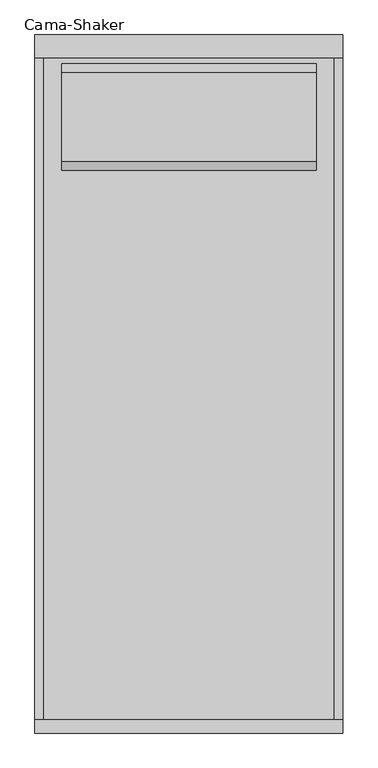
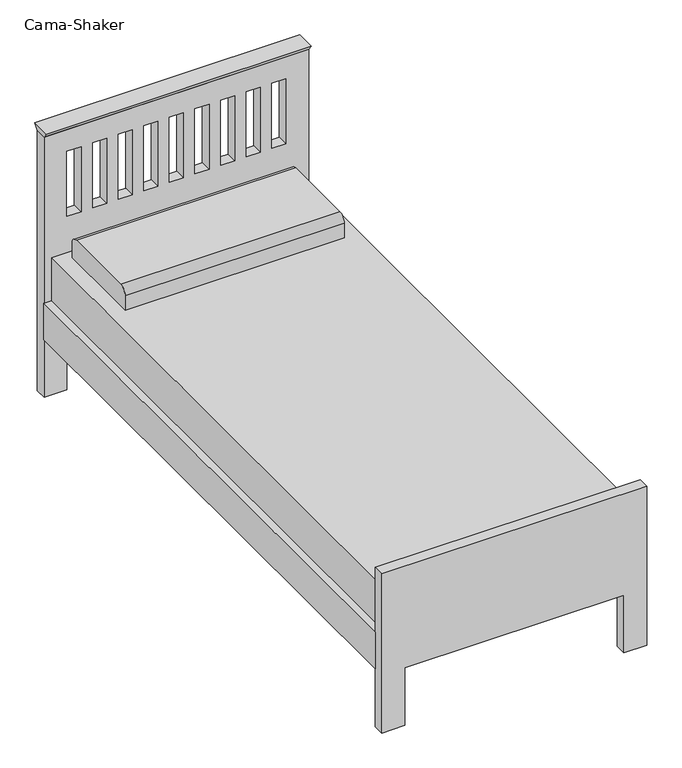
"""IFC4 building model written with IfcOpenShell, lengths in millimetres: furniture geometry, Cama-Shaker : 880 x 1981 mm - Solteiro."""

from ifc_helpers import new_model, si_unit, point, frame, frame_2d, origin, place, context, project, spatial, polyline, circle_curve, trimmed, segment, composite_curve, outline, extrude, source, transform, mapped, element, save


def cama_shaker_bda1b693(model_context):
    return source(origin(), model_context, "Body", "SweptSolid", [
        extrude(outline(polyline([(-38.1, 914.4), (-51.9545455, 933.45), (13.8545455, 933.45), (0.0, 914.4), (-38.1, 914.4)])), frame((-458.8365546, 0.0, 0.0), z_axis=(1.0, 0.0, 0.0), x_axis=(0.0, 1.0, 0.0)), (0.0, 0.0, 1.0), 880.0533613),
        extrude(outline(composite_curve([segment(polyline([(-373.2486637, 482.6), (-373.2486637, 533.4)]), True, "CONTINUOUS"), segment(trimmed(circle_curve(frame_2d((-347.8486637, 533.4)), 25.4), [point((-373.2486637, 533.4))], [point((-347.8486637, 558.8))], False, "CARTESIAN"), True, "CONTINUOUS"), segment(polyline([(-347.8486637, 558.8), (-93.8486637, 558.8)]), True, "CONTINUOUS"), segment(trimmed(circle_curve(frame_2d((-93.8486637, 533.4)), 25.4), [point((-93.8486637, 558.8))], [point((-68.4486637, 533.4))], False, "CARTESIAN"), True, "CONTINUOUS"), segment(polyline([(-68.4486637, 533.4), (-68.4486637, 482.6), (-373.2486637, 482.6)]), True, "CONTINUOUS")], self_intersect=False)), frame((-382.85, 0.0, 0.0), z_axis=(1.0, 0.0, 0.0), x_axis=(0.0, 1.0, 0.0)), (0.0, 0.0, 1.0), 727.6),
        extrude(outline(polyline([(395.55, -38.1), (395.55, -1943.1), (-433.65, -1943.1), (-433.65, -38.1), (395.55, -38.1)])), frame((0.0, 0.0, 228.6), z_axis=(0.0, 0.0, 1.0), x_axis=(1.0, 0.0, 0.0)), (0.0, 0.0, 1.0), 254.0),
        extrude(outline(polyline([(395.55, -1943.1), (395.55, -38.1), (420.95, -38.1), (420.95, -1943.1), (395.55, -1943.1)])), frame((0.0, 0.0, 203.0994861), z_axis=(0.0, 0.0, 1.0), x_axis=(1.0, 0.0, 0.0)), (0.0, 0.0, 1.0), 127.0),
        extrude(outline(polyline([(-459.05, -1943.1), (-459.05, -38.1), (-433.65, -38.1), (-433.65, -1943.1), (-459.05, -1943.1)])), frame((0.0, 0.0, 203.5755296), z_axis=(0.0, 0.0, 1.0), x_axis=(1.0, 0.0, 0.0)), (0.0, 0.0, 1.0), 127.0),
        extrude(outline(polyline([(0.0, -382.85), (203.2, -382.85), (203.2, 344.75), (0.0, 344.75), (0.0, 420.95), (558.8, 420.95), (558.8, -459.05), (0.0, -459.05), (0.0, -382.85)])), frame((0.0, -1981.2, 0.0), z_axis=(0.0, 1.0, 0.0), x_axis=(0.0, 0.0, 1.0)), (0.0, 0.0, 1.0), 38.1),
        extrude(outline(polyline([(914.4, 421.2168067), (914.4, -458.8365546), (0.0, -458.8365546), (0.0, -382.85), (203.2, -382.85), (203.2, 344.75), (0.0, 344.75), (0.0, 421.2168067), (914.4, 421.2168067)]), holes=[polyline([(838.2, -335.8722222), (609.6, -335.8722222), (609.6, -382.85), (838.2, -382.85), (838.2, -335.8722222)]), polyline([(838.2, -250.7944444), (609.6, -250.7944444), (609.6, -297.7722222), (838.2, -297.7722222), (838.2, -250.7944444)]), polyline([(838.2, -165.7166667), (609.6, -165.7166667), (609.6, -212.6944444), (838.2, -212.6944444), (838.2, -165.7166667)]), polyline([(838.2, -80.6388889), (609.6, -80.6388889), (609.6, -127.6166667), (838.2, -127.6166667), (838.2, -80.6388889)]), polyline([(838.2, 89.5166667), (609.6, 89.5166667), (609.6, 42.5388889), (838.2, 42.5388889), (838.2, 89.5166667)]), polyline([(838.2, 174.5944444), (609.6, 174.5944444), (609.6, 127.6166667), (838.2, 127.6166667), (838.2, 174.5944444)]), polyline([(838.2, 259.6722222), (609.6, 259.6722222), (609.6, 212.6944444), (838.2, 212.6944444), (838.2, 259.6722222)]), polyline([(838.2, 344.75), (609.6, 344.75), (609.6, 297.7722222), (838.2, 297.7722222), (838.2, 344.75)]), polyline([(838.2, 4.4388889), (609.6, 4.4388889), (609.6, -42.5388889), (838.2, -42.5388889), (838.2, 4.4388889)])]), frame((0.0, -38.1, 0.0), z_axis=(0.0, 1.0, 0.0), x_axis=(0.0, 0.0, 1.0)), (0.0, 0.0, 1.0), 38.1),
    ])


if __name__ == "__main__":
    model = new_model("IFC4")
    model_context = context("Model", 3, world=origin())
    ifc_project = project(units=[si_unit("LENGTHUNIT", "METRE", prefix="MILLI")], contexts=[model_context])
    site = spatial("IfcSite", under=ifc_project)
    building = spatial("IfcBuilding", under=site)
    placement = place(None, origin())
    cama_shaker_shape = cama_shaker_bda1b693(model_context)
    element("IfcFurniture", 1, ObjectType="Cama-Shaker : 880 x 1981 mm - Solteiro", at=placement, inside=building, context=model_context, shape_type="MappedRepresentation", body=[
        mapped(cama_shaker_shape, transform((0.0, 0.0, 0.0), x_axis=(1.0, 0.0, 0.0), y_axis=(0.0, 1.0, 0.0), z_axis=(0.0, 0.0, 1.0))),
    ])
    save(model, "model.ifc")

# Revit data of these elements
# Type "Cama-Shaker : 880 x 1981 mm - Solteiro"
#   Comprimento = 1.9812 m
#   Largura = 0.88 m
#   Material da moldura = wood brown
#   Material do colchão = Linho, branco
#   Default Elevation = 0
# Element 1 (IfcFurniture, "Cama-Shaker : 880 x 1981 mm - Solteiro")
#   Materials on its faces: "wood brown", "Linho, branco"
# Materials
#   "wood brown": class "Wood", colour RGB 80 39 12, transparency 0, Cost = 0
#   "Linho, branco": class "Tecido", colour RGB 247 247 239, transparency 0, Description = "Linho, branco", Cost = 0
